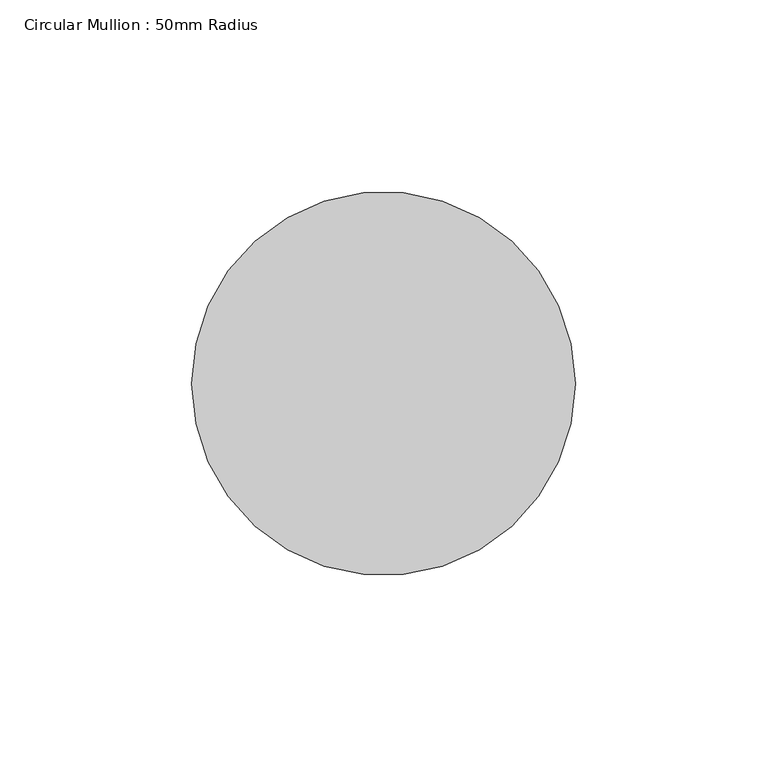
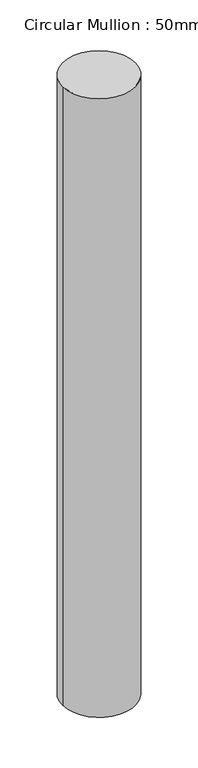
"""IFC4 building model written with IfcOpenShell, lengths in millimetres: member geometry, Circular Mullion : 50mm Radius."""

from ifc_helpers import new_model, si_unit, point, frame, origin, origin_2d, place, context, project, spatial, circle_curve, trimmed, segment, composite_curve, outline, extrude, source, transform, mapped, element, save


def circular_mullion_50mm_radius_0894eb31(model_context):
    return source(origin(), model_context, "Body", "SweptSolid", [
        extrude(outline(composite_curve([segment(trimmed(circle_curve(origin_2d(), 50.0), [point((50.0, 0.0))], [point((-50.0, 0.0))], False, "CARTESIAN"), True, "CONTINUOUS"), segment(trimmed(circle_curve(origin_2d(), 50.0), [point((-50.0, 0.0))], [point((50.0, 0.0))], False, "CARTESIAN"), True, "CONTINUOUS")], self_intersect=False)), frame((0.0, 0.0, -903.0397298), z_axis=(0.0, 0.0, 1.0), x_axis=(1.0, 0.0, 0.0)), (0.0, 0.0, 1.0), 903.0397298),
    ])


if __name__ == "__main__":
    model = new_model("IFC4")
    model_context = context("Model", 3, world=origin())
    ifc_project = project(units=[si_unit("LENGTHUNIT", "METRE", prefix="MILLI")], contexts=[model_context])
    site = spatial("IfcSite", under=ifc_project)
    building = spatial("IfcBuilding", under=site)
    placement = place(None, origin())
    circular_mullion_50mm_radius_shape = circular_mullion_50mm_radius_0894eb31(model_context)
    element("IfcMember", 1, ObjectType="Circular Mullion : 50mm Radius", at=placement, inside=building, context=model_context, shape_type="MappedRepresentation", body=[
        mapped(circular_mullion_50mm_radius_shape, transform((0.0, 0.0, 0.0), x_axis=(1.0, 0.0, 0.0), y_axis=(0.0, 1.0, 0.0), z_axis=(0.0, 0.0, 1.0))),
    ])
    save(model, "model.ifc")

# Revit data of these elements
# Type "Circular Mullion : 50mm Radius"
#   built-in parameter 1007350 = 0.164042 (stored number, unit not read)
# Element 1 (IfcMember, "Circular Mullion : 50mm Radius")
#   Materials on its faces: "Aluminium"
# Materials
#   "Aluminium": class "Metal", colour RGB 247 247 247, transparency 0, Description = "Aluminium 6061", Cost = 0
